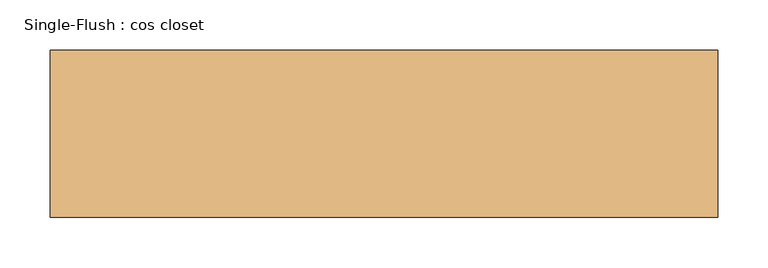
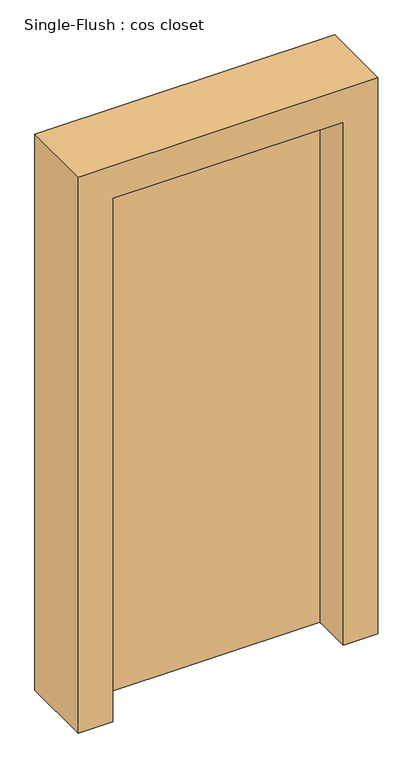
"""IFC4 building model written with IfcOpenShell, lengths in millimetres: door geometry, Single-Flush : cos closet."""

import ifcopenshell
import ifcopenshell.guid

model = None  # the IFC model being written
_history = None  # IfcOwnerHistory: only IFC2X3 demands one
_inside = {}  # id of a spatial element -> (the spatial element, [elements in it])
_under = {}  # id of a project, library or spatial element -> (it, [spatial elements below it])
_declared = {}  # id of a project -> (the project, [libraries it declares])
_typed = {}  # id of a type object -> (the type object, [elements of that type])
_made_of = {}  # id of a material, layer set ... -> (it, [elements and type objects made of it])


def new_model(schema):
    """Start an empty IFC model of exactly this schema.

    Asked for "IFC4X3", IfcOpenShell would pick the latest addendum, in which some entities
    have other attributes; the version numbers below select the first issue.
    IFC2X3 requires an IfcOwnerHistory on every rooted entity: one is made here for all.
    """
    global model, _history
    if schema == "IFC4X3":
        model = ifcopenshell.file(schema_version=(4, 3, 0, 0))
    else:
        model = ifcopenshell.file(schema=schema)
    _inside.clear()
    _under.clear()
    _declared.clear()
    _typed.clear()
    _made_of.clear()
    _history = None
    if model.schema == "IFC2X3":
        org = make("IfcOrganization", Name="unknown")
        user = make(
            "IfcPersonAndOrganization",
            ThePerson=make("IfcPerson", FamilyName="unknown"),
            TheOrganization=org,
        )
        app = make(
            "IfcApplication",
            ApplicationDeveloper=org,
            Version="unknown",
            ApplicationFullName="unknown",
            ApplicationIdentifier="unknown",
        )
        _history = make(
            "IfcOwnerHistory",
            OwningUser=user,
            OwningApplication=app,
            ChangeAction="ADDED",
            CreationDate=0,
        )
    return model


def make(cls, **values):
    """One entity of the class cls with the attributes given. An attribute that is None is left unset."""
    return model.create_entity(
        cls, **{name: value for name, value in values.items() if value is not None}
    )


def rooted(cls, **values):
    """An entity with a GlobalId (a new one), such as an element, a storey or a relation."""
    return make(cls, GlobalId=ifcopenshell.guid.new(), OwnerHistory=_history, **values)


def si_unit(unit_type, name, prefix=None):
    """IfcSIUnit, for example si_unit("LENGTHUNIT", "METRE", prefix="MILLI")."""
    return make("IfcSIUnit", UnitType=unit_type, Prefix=prefix, Name=name)


def assignment(units):
    """IfcUnitAssignment: the units of a project."""
    return None if units is None else make("IfcUnitAssignment", Units=units)


def point(xyz):
    """IfcCartesianPoint."""
    return None if xyz is None else make("IfcCartesianPoint", Coordinates=xyz)


def direction(xyz):
    """IfcDirection."""
    return None if xyz is None else make("IfcDirection", DirectionRatios=xyz)


def frame(location, z_axis=None, x_axis=None):
    """IfcAxis2Placement3D, a coordinate frame: its origin and axes. An axis left out is left unset."""
    return make(
        "IfcAxis2Placement3D",
        Location=point(location),
        Axis=direction(z_axis),
        RefDirection=direction(x_axis),
    )


def origin():
    """The frame at (0, 0, 0) with its axes left unset."""
    return frame((0.0, 0.0, 0.0))


def origin_with_axes():
    """The frame at (0, 0, 0) with the z axis (0, 0, 1) and the x axis (1, 0, 0) written out."""
    return frame((0.0, 0.0, 0.0), z_axis=(0.0, 0.0, 1.0), x_axis=(1.0, 0.0, 0.0))


def place(relative_to, where):
    """IfcLocalPlacement: puts the frame where relative to a parent placement (None: the world)."""
    return make(
        "IfcLocalPlacement", PlacementRelTo=relative_to, RelativePlacement=where
    )


def context(
    kind, dimensions, precision=None, world=None, true_north=None, identifier=None
):
    """IfcGeometricRepresentationContext, for example the 3D "Model" context."""
    return make(
        "IfcGeometricRepresentationContext",
        ContextIdentifier=identifier,
        ContextType=kind,
        CoordinateSpaceDimension=dimensions,
        Precision=precision,
        WorldCoordinateSystem=world,
        TrueNorth=true_north,
    )


def project(units=None, contexts=None):
    """IfcProject with its units and contexts."""
    return rooted(
        "IfcProject",
        Name="project",
        RepresentationContexts=contexts,
        UnitsInContext=assignment(units),
    )


def spatial(cls, under=None, at=None, **own):
    """A site, building, storey or space (cls), placed at a placement, below another one or the project."""
    s = rooted(cls, ObjectPlacement=at, **own)
    if under is not None:
        _under.setdefault(under.id(), (under, []))[1].append(s)
    return s


def polyline(points):
    """IfcPolyline through the points."""
    return make("IfcPolyline", Points=[point(p) for p in points])


def outline(outer, holes=None, kind="AREA"):
    """IfcArbitraryClosedProfileDef: a profile drawn as a closed curve; with holes, ...WithVoids."""
    if holes is None:
        return make("IfcArbitraryClosedProfileDef", ProfileType=kind, OuterCurve=outer)
    return make(
        "IfcArbitraryProfileDefWithVoids",
        ProfileType=kind,
        OuterCurve=outer,
        InnerCurves=holes,
    )


def extrude(swept, where, along, depth):
    """IfcExtrudedAreaSolid: the profile swept, set in the frame where, extruded along a direction by depth."""
    return make(
        "IfcExtrudedAreaSolid",
        SweptArea=swept,
        Position=where,
        ExtrudedDirection=direction(along),
        Depth=depth,
    )


def shape(context_of_items, identifier, shape_type, items):
    """IfcShapeRepresentation: the items that make up one representation, for example the "Body"."""
    return make(
        "IfcShapeRepresentation",
        ContextOfItems=context_of_items,
        RepresentationIdentifier=identifier,
        RepresentationType=shape_type,
        Items=items,
    )


def source(mapping_origin, context_of_items, identifier, shape_type, items):
    """IfcRepresentationMap: a shape defined once, which mapped items show again and again."""
    return make(
        "IfcRepresentationMap",
        MappingOrigin=mapping_origin,
        MappedRepresentation=shape(context_of_items, identifier, shape_type, items),
    )


def transform(
    local_origin,
    x_axis=None,
    y_axis=None,
    z_axis=None,
    scale=None,
    scale2=None,
    scale3=None,
    uniform=True,
):
    """IfcCartesianTransformationOperator3D, or its non-uniform kind. x_axis, y_axis, z_axis: its Axis1, 2, 3."""
    if uniform:
        return make(
            "IfcCartesianTransformationOperator3D",
            Axis1=direction(x_axis),
            Axis2=direction(y_axis),
            LocalOrigin=point(local_origin),
            Scale=scale,
            Axis3=direction(z_axis),
        )
    return make(
        "IfcCartesianTransformationOperator3DnonUniform",
        Axis1=direction(x_axis),
        Axis2=direction(y_axis),
        LocalOrigin=point(local_origin),
        Scale=scale,
        Axis3=direction(z_axis),
        Scale2=scale2,
        Scale3=scale3,
    )


def mapped(mapping_source, mapping_target):
    """IfcMappedItem: shows the shape of a source again, moved by a transform."""
    return make(
        "IfcMappedItem", MappingSource=mapping_source, MappingTarget=mapping_target
    )


def made_of(thing, what):
    """Note that an element or type object is made of a material, layer set ...; save() writes the relation."""
    if what is not None:
        _made_of.setdefault(what.id(), (what, []))[1].append(thing)
    return thing


def element(
    cls,
    number,
    at=None,
    inside=None,
    cuts=None,
    type_object=None,
    material=None,
    context=None,
    identifier="Body",
    shape_type=None,
    held_by="IfcProductDefinitionShape",
    body=None,
    shapes=None,
    **own,
):
    """One element of the class cls, such as IfcWall. Its Tag is "e" and its number.

    at: its placement. inside: the storey or other place that contains it. cuts: it is an
    opening in that element (IfcRelVoidsElement). A single representation is given by context,
    identifier, shape_type and body (its items); several are given by shapes. held_by: the class
    of the entity that holds the representations. save() writes the other relations.
    """
    e = rooted(cls, Tag="e%d" % number, ObjectPlacement=at, **own)
    if body is not None:
        shapes = [shape(context, identifier, shape_type, body)]
    if shapes is not None:
        e.Representation = make(held_by, Representations=shapes)
    if inside is not None:
        _inside.setdefault(inside.id(), (inside, []))[1].append(e)
    if cuts is not None:
        rooted(
            "IfcRelVoidsElement", RelatingBuildingElement=cuts, RelatedOpeningElement=e
        )
    if type_object is not None:
        _typed.setdefault(type_object.id(), (type_object, []))[1].append(e)
    return made_of(e, material)


def aggregate(whole, parts):
    """IfcRelAggregates: a whole, such as a stair, and the parts it consists of."""
    return rooted("IfcRelAggregates", RelatingObject=whole, RelatedObjects=parts)


def save(model, path):
    """Write the relations noted so far, then the file.

    IfcRelAggregates (storeys below a building ...), IfcRelContainedInSpatialStructure (elements
    in a storey), IfcRelDefinesByType, IfcRelAssociatesMaterial and IfcRelDeclares: one each for
    every whole, place, type object, material and project.
    """
    for whole, parts in _under.values():
        aggregate(whole, parts)
    for where, things in _inside.values():
        rooted(
            "IfcRelContainedInSpatialStructure",
            RelatedElements=things,
            RelatingStructure=where,
        )
    for kind, things in _typed.values():
        rooted("IfcRelDefinesByType", RelatedObjects=things, RelatingType=kind)
    for what, things in _made_of.values():
        rooted("IfcRelAssociatesMaterial", RelatedObjects=things, RelatingMaterial=what)
    for by, libraries in _declared.values():
        rooted("IfcRelDeclares", RelatingContext=by, RelatedDefinitions=libraries)
    model.write(path)


def single_flush_cos_closet_870e594d(model_context):
    return source(origin(), model_context, "Body", "SweptSolid", [
        extrude(outline(polyline([(1295.4, 330.2), (1295.4, -330.2), (0.0, -330.2), (0.0, -254.0), (1219.2, -254.0), (1219.2, 254.0), (0.0, 254.0), (0.0, 330.2), (1295.4, 330.2)])), frame((0.0, -82.55, 0.0), z_axis=(0.0, 1.0, 0.0), x_axis=(0.0, 0.0, 1.0)), (0.0, 0.0, 1.0), 165.1),
        extrude(outline(polyline([(254.0, 6.35), (-254.0, 6.35), (-254.0, 57.15), (254.0, 57.15), (254.0, 6.35)])), origin_with_axes(), (0.0, 0.0, 1.0), 1219.2),
    ])


if __name__ == "__main__":
    model = new_model("IFC4")
    model_context = context("Model", 3, world=origin())
    ifc_project = project(units=[si_unit("LENGTHUNIT", "METRE", prefix="MILLI")], contexts=[model_context])
    site = spatial("IfcSite", under=ifc_project)
    building = spatial("IfcBuilding", under=site)
    placement = place(None, origin())
    single_flush_cos_closet_shape = single_flush_cos_closet_870e594d(model_context)
    element("IfcDoor", 1, ObjectType="Single-Flush : cos closet", at=placement, inside=building, context=model_context, shape_type="MappedRepresentation", body=[
        mapped(single_flush_cos_closet_shape, transform((0.0, 0.0, 0.0), x_axis=(1.0, 0.0, 0.0), y_axis=(0.0, 1.0, 0.0), z_axis=(0.0, 0.0, 1.0))),
    ])
    save(model, "model.ifc")

# Revit data of these elements
# Type "Single-Flush : cos closet"
#   Type Mark = "68"
#   OD_DS_Door_Material = "T.B.D."
#   OD_DS_Door_Type = "SWING"
#   OD_DS_Lockset = "PRIVACY LOCK"
#   Assembly Code = "C1020"
#   Analytic Construction = "<None>"
#   Thickness = 0' - 2"
#   RO Offset = 0' - 0 1/4"
#   Height = 4' - 0"
#   Trim Projection Ext = 0' - 1"
#   Trim Projection Int = 0' - 1"
#   Trim Width = 0' - 3"
#   Width = 1' - 8"
#   Door Material = Closet_1
#   Frame Material = Closet_1
#   Function = (empty or 0)
#   Wall Closure = (empty or 0)
# Element 1 (IfcDoor, "Single-Flush : cos closet")
#   Materials on its faces: "Closet_1"
# Materials
#   "Closet_1": class "Paint", colour RGB 200 194 183, transparency 0, Cost = 0
